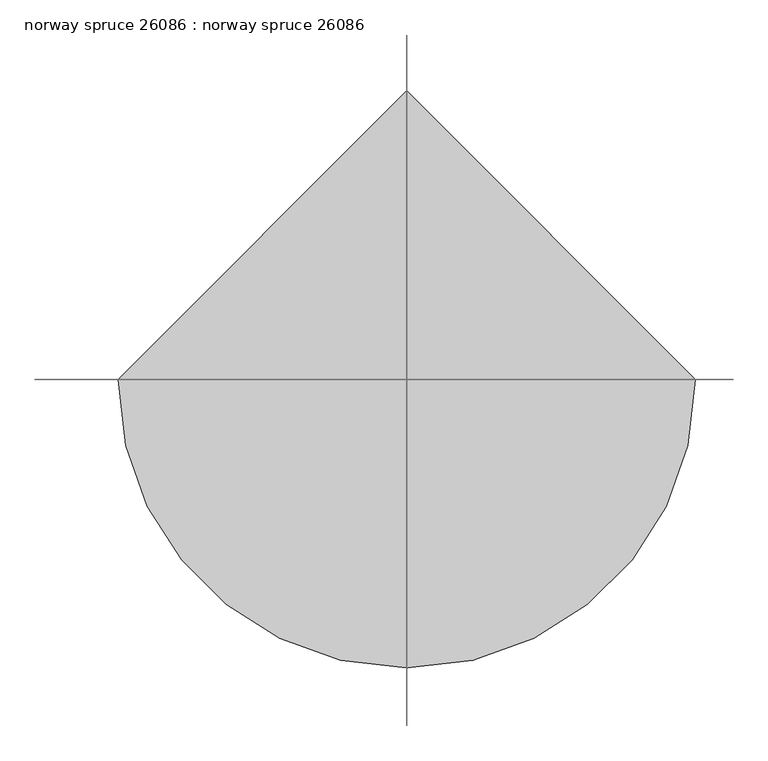
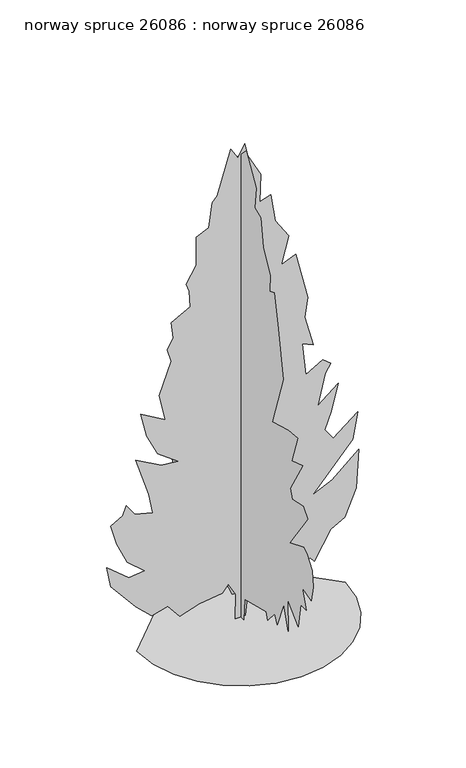
"""IFC4 building model written with IfcOpenShell, lengths in millimetres: proxy geometry, norway spruce 26086 : norway spruce 26086."""

import ifcopenshell
import ifcopenshell.guid

model = None  # the IFC model being written
_history = None  # IfcOwnerHistory: only IFC2X3 demands one
_inside = {}  # id of a spatial element -> (the spatial element, [elements in it])
_under = {}  # id of a project, library or spatial element -> (it, [spatial elements below it])
_declared = {}  # id of a project -> (the project, [libraries it declares])
_typed = {}  # id of a type object -> (the type object, [elements of that type])
_made_of = {}  # id of a material, layer set ... -> (it, [elements and type objects made of it])


def new_model(schema):
    """Start an empty IFC model of exactly this schema.

    Asked for "IFC4X3", IfcOpenShell would pick the latest addendum, in which some entities
    have other attributes; the version numbers below select the first issue.
    IFC2X3 requires an IfcOwnerHistory on every rooted entity: one is made here for all.
    """
    global model, _history
    if schema == "IFC4X3":
        model = ifcopenshell.file(schema_version=(4, 3, 0, 0))
    else:
        model = ifcopenshell.file(schema=schema)
    _inside.clear()
    _under.clear()
    _declared.clear()
    _typed.clear()
    _made_of.clear()
    _history = None
    if model.schema == "IFC2X3":
        org = make("IfcOrganization", Name="unknown")
        user = make(
            "IfcPersonAndOrganization",
            ThePerson=make("IfcPerson", FamilyName="unknown"),
            TheOrganization=org,
        )
        app = make(
            "IfcApplication",
            ApplicationDeveloper=org,
            Version="unknown",
            ApplicationFullName="unknown",
            ApplicationIdentifier="unknown",
        )
        _history = make(
            "IfcOwnerHistory",
            OwningUser=user,
            OwningApplication=app,
            ChangeAction="ADDED",
            CreationDate=0,
        )
    return model


def make(cls, **values):
    """One entity of the class cls with the attributes given. An attribute that is None is left unset."""
    return model.create_entity(
        cls, **{name: value for name, value in values.items() if value is not None}
    )


def rooted(cls, **values):
    """An entity with a GlobalId (a new one), such as an element, a storey or a relation."""
    return make(cls, GlobalId=ifcopenshell.guid.new(), OwnerHistory=_history, **values)


def si_unit(unit_type, name, prefix=None):
    """IfcSIUnit, for example si_unit("LENGTHUNIT", "METRE", prefix="MILLI")."""
    return make("IfcSIUnit", UnitType=unit_type, Prefix=prefix, Name=name)


def assignment(units):
    """IfcUnitAssignment: the units of a project."""
    return None if units is None else make("IfcUnitAssignment", Units=units)


def point(xyz):
    """IfcCartesianPoint."""
    return None if xyz is None else make("IfcCartesianPoint", Coordinates=xyz)


def direction(xyz):
    """IfcDirection."""
    return None if xyz is None else make("IfcDirection", DirectionRatios=xyz)


def frame(location, z_axis=None, x_axis=None):
    """IfcAxis2Placement3D, a coordinate frame: its origin and axes. An axis left out is left unset."""
    return make(
        "IfcAxis2Placement3D",
        Location=point(location),
        Axis=direction(z_axis),
        RefDirection=direction(x_axis),
    )


def origin():
    """The frame at (0, 0, 0) with its axes left unset."""
    return frame((0.0, 0.0, 0.0))


def place(relative_to, where):
    """IfcLocalPlacement: puts the frame where relative to a parent placement (None: the world)."""
    return make(
        "IfcLocalPlacement", PlacementRelTo=relative_to, RelativePlacement=where
    )


def context(
    kind, dimensions, precision=None, world=None, true_north=None, identifier=None
):
    """IfcGeometricRepresentationContext, for example the 3D "Model" context."""
    return make(
        "IfcGeometricRepresentationContext",
        ContextIdentifier=identifier,
        ContextType=kind,
        CoordinateSpaceDimension=dimensions,
        Precision=precision,
        WorldCoordinateSystem=world,
        TrueNorth=true_north,
    )


def project(units=None, contexts=None):
    """IfcProject with its units and contexts."""
    return rooted(
        "IfcProject",
        Name="project",
        RepresentationContexts=contexts,
        UnitsInContext=assignment(units),
    )


def spatial(cls, under=None, at=None, **own):
    """A site, building, storey or space (cls), placed at a placement, below another one or the project."""
    s = rooted(cls, ObjectPlacement=at, **own)
    if under is not None:
        _under.setdefault(under.id(), (under, []))[1].append(s)
    return s


def point_list(points):
    """IfcCartesianPointList2D or 3D."""
    cls = (
        "IfcCartesianPointList2D" if len(points[0]) == 2 else "IfcCartesianPointList3D"
    )
    return make(cls, CoordList=points)


def triangles(points, corners, closed=None, point_numbers=None):
    """IfcTriangulatedFaceSet: each triangle names its three corners, points numbered from 1."""
    return make(
        "IfcTriangulatedFaceSet",
        Coordinates=point_list(points),
        Closed=closed,
        CoordIndex=corners,
        PnIndex=point_numbers,
    )


def shape(context_of_items, identifier, shape_type, items):
    """IfcShapeRepresentation: the items that make up one representation, for example the "Body"."""
    return make(
        "IfcShapeRepresentation",
        ContextOfItems=context_of_items,
        RepresentationIdentifier=identifier,
        RepresentationType=shape_type,
        Items=items,
    )


def source(mapping_origin, context_of_items, identifier, shape_type, items):
    """IfcRepresentationMap: a shape defined once, which mapped items show again and again."""
    return make(
        "IfcRepresentationMap",
        MappingOrigin=mapping_origin,
        MappedRepresentation=shape(context_of_items, identifier, shape_type, items),
    )


def transform(
    local_origin,
    x_axis=None,
    y_axis=None,
    z_axis=None,
    scale=None,
    scale2=None,
    scale3=None,
    uniform=True,
):
    """IfcCartesianTransformationOperator3D, or its non-uniform kind. x_axis, y_axis, z_axis: its Axis1, 2, 3."""
    if uniform:
        return make(
            "IfcCartesianTransformationOperator3D",
            Axis1=direction(x_axis),
            Axis2=direction(y_axis),
            LocalOrigin=point(local_origin),
            Scale=scale,
            Axis3=direction(z_axis),
        )
    return make(
        "IfcCartesianTransformationOperator3DnonUniform",
        Axis1=direction(x_axis),
        Axis2=direction(y_axis),
        LocalOrigin=point(local_origin),
        Scale=scale,
        Axis3=direction(z_axis),
        Scale2=scale2,
        Scale3=scale3,
    )


def mapped(mapping_source, mapping_target):
    """IfcMappedItem: shows the shape of a source again, moved by a transform."""
    return make(
        "IfcMappedItem", MappingSource=mapping_source, MappingTarget=mapping_target
    )


def made_of(thing, what):
    """Note that an element or type object is made of a material, layer set ...; save() writes the relation."""
    if what is not None:
        _made_of.setdefault(what.id(), (what, []))[1].append(thing)
    return thing


def element(
    cls,
    number,
    at=None,
    inside=None,
    cuts=None,
    type_object=None,
    material=None,
    context=None,
    identifier="Body",
    shape_type=None,
    held_by="IfcProductDefinitionShape",
    body=None,
    shapes=None,
    **own,
):
    """One element of the class cls, such as IfcWall. Its Tag is "e" and its number.

    at: its placement. inside: the storey or other place that contains it. cuts: it is an
    opening in that element (IfcRelVoidsElement). A single representation is given by context,
    identifier, shape_type and body (its items); several are given by shapes. held_by: the class
    of the entity that holds the representations. save() writes the other relations.
    """
    e = rooted(cls, Tag="e%d" % number, ObjectPlacement=at, **own)
    if body is not None:
        shapes = [shape(context, identifier, shape_type, body)]
    if shapes is not None:
        e.Representation = make(held_by, Representations=shapes)
    if inside is not None:
        _inside.setdefault(inside.id(), (inside, []))[1].append(e)
    if cuts is not None:
        rooted(
            "IfcRelVoidsElement", RelatingBuildingElement=cuts, RelatedOpeningElement=e
        )
    if type_object is not None:
        _typed.setdefault(type_object.id(), (type_object, []))[1].append(e)
    return made_of(e, material)


def aggregate(whole, parts):
    """IfcRelAggregates: a whole, such as a stair, and the parts it consists of."""
    return rooted("IfcRelAggregates", RelatingObject=whole, RelatedObjects=parts)


def save(model, path):
    """Write the relations noted so far, then the file.

    IfcRelAggregates (storeys below a building ...), IfcRelContainedInSpatialStructure (elements
    in a storey), IfcRelDefinesByType, IfcRelAssociatesMaterial and IfcRelDeclares: one each for
    every whole, place, type object, material and project.
    """
    for whole, parts in _under.values():
        aggregate(whole, parts)
    for where, things in _inside.values():
        rooted(
            "IfcRelContainedInSpatialStructure",
            RelatedElements=things,
            RelatingStructure=where,
        )
    for kind, things in _typed.values():
        rooted("IfcRelDefinesByType", RelatedObjects=things, RelatingType=kind)
    for what, things in _made_of.values():
        rooted("IfcRelAssociatesMaterial", RelatedObjects=things, RelatingMaterial=what)
    for by, libraries in _declared.values():
        rooted("IfcRelDeclares", RelatingContext=by, RelatedDefinitions=libraries)
    model.write(path)


def norway_spruce_26086_norway_spruce_26086_64d82020(model_context):
    return source(origin(), model_context, "Body", "Tessellation", [
        triangles([(-954.9721601, 0.0, 2.42e-05), (-929.7245733, -218.8163494, 2.42e-05), (-857.8247469, -419.7632589, 2.42e-05), (-745.0257454, -597.0859019, 2.42e-05), (-597.0859019, -745.0257454, 2.42e-05), (-419.7632589, -857.8247469, 2.42e-05), (-218.816095, -929.7245733, 2.42e-05), (4.17e-05, -954.9721601, 2.42e-05), (218.8163494, -929.7245733, 2.42e-05), (419.7632589, -857.8247469, 2.42e-05), (597.0859019, -745.0257454, 2.42e-05), (745.0257454, -597.0859019, 2.42e-05), (857.8247469, -419.7632589, 2.42e-05), (929.7245733, -218.816095, 2.42e-05), (954.9721601, 8.35e-05, 2.42e-05), (-0.0001252, 954.9721601, 2.42e-05), (-52.0131451, 2.3e-06, 4.1e-06), (-45.7469624, -1.19e-05, 233.9905685), (-114.4303972, -1.64e-05, 358.8946632), (-169.0439877, -9.8e-06, 288.6763112), (-379.1994558, 1.2e-06, 258.1937423), (-559.1458849, 1.24e-05, 202.8534611), (-668.3761362, 9.2e-06, 335.4885338), (-816.615707, 1.8e-05, 296.4791961), (-964.852807, 1.61e-05, 436.9159184), (-1191.113633, 9.7e-06, 709.9864597), (-1230.1230251, -2e-07, 905.0382895), (-1027.2707994, 7e-07, 741.1954559), (-879.0312286, -6.7e-06, 756.7987186), (-1042.8740622, -7.9e-06, 897.2354227), (-1136.4985073, -1.59e-05, 1100.0901192), (-1191.113633, -2.51e-05, 1295.1420216), (-1081.8833817, -3.36e-05, 1357.5573978), (-1050.6769289, -4.01e-05, 1443.3790489), (-972.6556738, -3.7e-05, 1334.1512684), (-808.8128403, -4.18e-05, 1295.1420216), (-842.6787237, -5.17e-05, 1484.6641743), (-964.852807, -6.85e-05, 1856.8888378), (-730.7915852, -7.08e-05, 1724.252457), (-574.2893646, -7.68e-05, 1709.7591557), (-762.0005814, -7.69e-05, 1849.0859711), (-863.4279659, -8.46e-05, 2051.9405949), (-918.0405481, -9.61e-05, 2286.0018894), (-691.7822657, -9.81e-05, 2153.3655087), (-746.3948479, -0.0001106, 2403.0323914), (-637.16714, -0.0001331, 2699.5142944), (-676.1764595, -0.0001388, 2824.3552208), (-621.5638773, -0.0001472, 2925.7775185), (-637.16714, -0.0001554, 3074.012075), (-465.5214034, -0.0001685, 3167.6365929), (-473.7865966, -0.0001773, 3322.3989487), (-501.9145672, -0.0001809, 3402.2818634), (-410.9062778, -0.0001936, 3549.9321533), (-410.9062778, -0.0002099, 3823.0079269), (-295.541935, -0.000218, 3874.3158417), (-262.6692322, -0.0002331, 4103.8811897), (-215.8559741, -0.0002384, 4158.4912285), (-91.0235138, -0.0002681, 4564.2057083), (-28.607027, -0.0002648, 4462.7837013), (33.8094597, -0.000274, 4572.0037788), (65.0179563, -0.0002679, 4447.1625618), (182.0485537, -0.00026, 4228.7224068), (174.2464318, -0.0002439, 3963.4447037), (275.6715091, -0.0002501, 3994.6611122), (314.6834084, -0.000236, 3729.3834091), (439.516886, -0.0002303, 3542.1343735), (369.2984977, -0.0002119, 3284.6544502), (501.932335, -0.000221, 3339.2897781), (611.1626226, -0.0001988, 2886.7630394), (587.7564569, -0.0001866, 2699.5142944), (665.7752048, -0.0001723, 2403.0323914), (564.3503637, -0.0001707, 2449.8446503), (595.5568165, -0.0001535, 2137.7622459), (751.5993267, -0.0001659, 2231.3867638), (821.8176424, -0.0001652, 2168.9712421), (775.0054562, -0.0001585, 2090.949987), (704.7870678, -0.0001382, 1802.2737122), (892.0360308, -0.0001553, 1950.5132103), (829.6180384, -0.0001376, 1700.8487984), (767.2025167, -0.0001256, 1544.8064335), (845.2237719, -0.0001225, 1435.578653), (1071.4820543, -0.0001431, 1615.0246765), (1024.6698681, -0.0001262, 1365.3602646), (657.9748089, -8.55e-05, 951.8505484), (837.4209051, -9.85e-05, 1037.6721268), (1079.3611519, -0.0001214, 1245.4696175), (1055.8788643, -9.87e-05, 881.63216), (954.4514797, -7.94e-05, 631.9652046), (821.8176424, -6.94e-05, 561.7468526), (673.5780716, -4.76e-05, 304.2795376), (634.5686794, -4.87e-05, 351.0917965), (369.2984977, -2.4e-05, 132.6348456), (345.8924046, -2.91e-05, 234.0616942), (135.2360586, -1.47e-05, 148.2390894), (65.017702, -1.54e-05, 210.6553286), (41.6113273, -1.8e-06, 0.0), (2.1e-06, 47.3113473, 2.84e-05), (8.7e-06, 70.7174676, 187.2491992), (1.01e-05, 133.1339521, 140.4369675), (1.64e-05, 242.3629317, 187.2491992), (2.32e-05, 382.7986184, 202.8534611), (3.05e-05, 546.6439954, 202.8534611), (3.7e-05, 587.3043406, 362.1915914), (4.1e-05, 710.7459337, 309.7887943), (4.73e-05, 772.9023142, 429.1130153), (6.07e-05, 952.3508812, 608.5590752), (7.81e-05, 1123.9941107, 936.2472857), (8.19e-05, 1139.5998442, 1037.6721268), (6.4e-05, 811.9116337, 928.4444189), (7.9e-05, 1006.9634634, 1139.0994387), (9.36e-05, 1119.7776529, 1460.6409313), (8.24e-05, 908.7847904, 1401.7661819), (8.72e-05, 905.5361515, 1568.2125629), (8.01e-05, 772.9023142, 1529.2031708), (8.81e-05, 827.5174398, 1716.4520611), (9.88e-05, 843.1206299, 2051.9405949), (8.05e-05, 515.4349992, 1927.1072262), (9.28e-05, 640.2684769, 2153.3679794), (0.0001013, 601.2565776, 2496.6569092), (0.0001109, 671.4749296, 2715.1098541), (0.0001132, 567.9546132, 2944.9036766), (0.0001197, 559.9028154, 3177.6441216), (0.0001155, 398.4043882, 3276.8566704), (0.0001214, 437.4137441, 3417.2934471), (0.0001235, 308.7626578, 3682.0124634), (0.0001285, 273.5709105, 3901.0365944), (0.0001262, 211.1544261, 3916.6324448), (0.0001321, 94.123588, 4291.1302254), (0.0001344, 62.9153412, 4415.9714424), (0.0001324, -85.3229897, 4572.0037788), (0.0001173, -241.3647005, 4298.9280052), (0.0001123, -217.9585892, 4096.0834099), (0.0001069, -319.3849382, 4064.8667107), (9.72e-05, -358.3968375, 3799.5890076), (8.63e-05, -467.6245454, 3596.7444122), (8.18e-05, -459.8216423, 3432.914296), (7.95e-05, -530.0399943, 3464.105706), (6.75e-05, -592.4580231, 3152.0410332), (5.07e-05, -670.4767347, 2707.3120743), (4.3e-05, -498.8335416, 2192.3773716), (3.4e-05, -749.4961847, 2265.5522655), (2.75e-05, -904.5378839, 2278.1988773), (2.35e-05, -810.9134388, 2005.128336), (1.75e-05, -982.5591391, 2059.7409908), (1.62e-05, -787.5073093, 1724.2549278), (1.22e-05, -818.7163055, 1638.430806), (5.5e-06, -992.5565666, 1672.3220512), (0.0, -1060.5803942, 1591.6185471), (7e-07, -779.706986, 1193.7145643), (-6.5e-06, -998.1649452, 1279.5361427), (-1.01e-05, -1052.7775274, 1240.5268959), (-1.68e-05, -1130.7987099, 1131.2965719), (-2.2e-05, -1146.4019726, 983.0595446), (-2.5e-05, -1115.1955198, 834.8199011), (-1.75e-05, -974.7588158, 873.8292933), (-2.57e-05, -1037.1742647, 694.383197), (-2.18e-05, -951.3526863, 694.383197), (-2.71e-05, -912.3408234, 460.3220115), (-1.47e-05, -740.6950504, 616.3619419), (-2.43e-05, -756.3008566, 319.8853074), (-1.45e-05, -678.2796015, 530.5403998), (-1.76e-05, -576.8522532, 273.0730848), (-1.33e-05, -537.8428974, 358.8946632), (-1.24e-05, -428.6126461, 226.2595724), (-9.3e-06, -405.2065166, 296.4791961), (3.5e-06, -61.9173734, 210.655583), (-2.1e-06, -46.3131251, 2.56e-05)], [[15, 16, 1], [14, 15, 1], [14, 1, 2], [13, 14, 2], [13, 2, 3], [13, 3, 4], [12, 13, 4], [11, 12, 4], [11, 4, 5], [11, 5, 6], [11, 6, 7], [11, 7, 8], [11, 8, 9], [11, 9, 10], [77, 78, 79], [81, 82, 83], [37, 38, 39], [59, 60, 61], [85, 86, 87], [42, 43, 44], [57, 58, 59], [70, 71, 72], [33, 34, 35], [91, 92, 93], [89, 90, 91], [81, 83, 84], [26, 27, 28], [25, 26, 28], [67, 68, 69], [63, 64, 65], [25, 28, 29], [96, 17, 18], [95, 96, 18], [41, 42, 44], [74, 75, 76], [73, 74, 76], [73, 76, 77], [85, 87, 88], [84, 85, 88], [84, 88, 89], [31, 32, 33], [31, 33, 35], [77, 79, 80], [37, 39, 40], [31, 35, 36], [30, 31, 36], [29, 30, 36], [21, 22, 23], [48, 49, 50], [40, 41, 44], [53, 54, 55], [84, 89, 91], [84, 91, 93], [93, 94, 95], [84, 93, 95], [84, 95, 18], [84, 18, 19], [24, 25, 29], [23, 24, 29], [36, 37, 40], [80, 81, 84], [59, 61, 62], [57, 59, 62], [57, 62, 63], [56, 57, 63], [55, 56, 63], [55, 63, 65], [53, 55, 65], [53, 65, 66], [53, 66, 67], [52, 53, 67], [51, 52, 67], [50, 51, 67], [50, 67, 69], [50, 69, 70], [48, 50, 70], [48, 70, 72], [47, 48, 72], [46, 47, 72], [45, 46, 72], [44, 45, 72], [44, 72, 73], [40, 44, 73], [40, 73, 77], [40, 77, 80], [40, 80, 84], [40, 84, 19], [36, 40, 19], [29, 36, 19], [23, 29, 19], [21, 23, 19], [20, 21, 19], [159, 160, 161], [143, 144, 145], [161, 162, 163], [110, 111, 112], [157, 158, 159], [163, 164, 165], [107, 108, 109], [106, 107, 109], [141, 142, 143], [115, 116, 117], [155, 156, 157], [129, 130, 131], [112, 113, 114], [136, 137, 138], [128, 129, 131], [128, 131, 132], [127, 128, 132], [153, 154, 155], [140, 141, 143], [166, 167, 97], [166, 97, 98], [103, 104, 105], [101, 102, 103], [147, 148, 149], [146, 147, 149], [114, 115, 117], [105, 106, 109], [125, 126, 127], [103, 105, 109], [132, 133, 134], [127, 132, 134], [125, 127, 134], [125, 134, 135], [125, 135, 136], [124, 125, 136], [123, 124, 136], [123, 136, 138], [123, 138, 139], [123, 139, 140], [122, 123, 140], [121, 122, 140], [120, 121, 140], [119, 120, 140], [118, 119, 140], [117, 118, 140], [140, 143, 145], [117, 140, 145], [114, 117, 145], [114, 145, 146], [114, 146, 149], [152, 153, 155], [151, 152, 155], [150, 151, 155], [149, 150, 155], [109, 110, 112], [155, 157, 159], [149, 155, 159], [114, 149, 159], [114, 159, 161], [114, 161, 163], [114, 163, 165], [114, 165, 166], [114, 166, 98], [112, 114, 98], [109, 112, 98], [103, 109, 98], [101, 103, 98], [100, 101, 98], [99, 100, 98]], closed=False),
    ])


if __name__ == "__main__":
    model = new_model("IFC4")
    model_context = context("Model", 3, world=origin())
    ifc_project = project(units=[si_unit("LENGTHUNIT", "METRE", prefix="MILLI")], contexts=[model_context])
    site = spatial("IfcSite", under=ifc_project)
    building = spatial("IfcBuilding", under=site)
    placement = place(None, origin())
    norway_spruce_26086_norway_spruce_26086_shape = norway_spruce_26086_norway_spruce_26086_64d82020(model_context)
    element("IfcBuildingElementProxy", 1, Name="norway spruce 26086 : norway spruce 26086", ObjectType="norway spruce 26086 : norway spruce 26086", at=placement, inside=building, context=model_context, shape_type="MappedRepresentation", body=[
        mapped(norway_spruce_26086_norway_spruce_26086_shape, transform((0.0, 0.0, 0.0), x_axis=(1.0, 0.0, 0.0), y_axis=(0.0, 1.0, 0.0), z_axis=(0.0, 0.0, 1.0))),
    ])
    save(model, "model.ifc")

# Revit data of these elements
# Type "norway spruce 26086 : norway spruce 26086"
#   built-in parameter 1005195 = "RPC-16-FXGW-0XFX-PJ97-W000-ST1L-LVER-AU"
#   Height = 0
